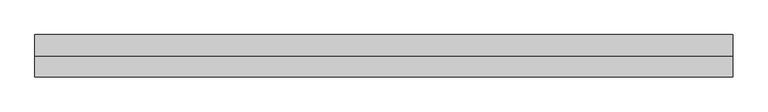
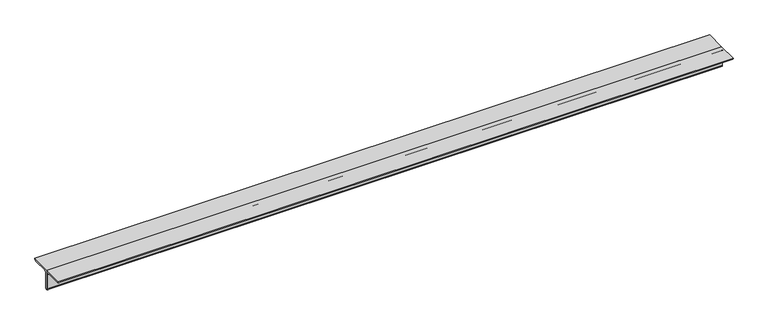
"""IFC4 building model written with IfcOpenShell, lengths in millimetres: member geometry, 0123_Steel Framing_2Ls-KSD3502 : H_SB_AR_S03_2Ls-130x130x12_HBR4."""

import ifcopenshell
import ifcopenshell.guid

model = None  # the IFC model being written
_history = None  # IfcOwnerHistory: only IFC2X3 demands one
_inside = {}  # id of a spatial element -> (the spatial element, [elements in it])
_under = {}  # id of a project, library or spatial element -> (it, [spatial elements below it])
_declared = {}  # id of a project -> (the project, [libraries it declares])
_typed = {}  # id of a type object -> (the type object, [elements of that type])
_made_of = {}  # id of a material, layer set ... -> (it, [elements and type objects made of it])


def new_model(schema):
    """Start an empty IFC model of exactly this schema.

    Asked for "IFC4X3", IfcOpenShell would pick the latest addendum, in which some entities
    have other attributes; the version numbers below select the first issue.
    IFC2X3 requires an IfcOwnerHistory on every rooted entity: one is made here for all.
    """
    global model, _history
    if schema == "IFC4X3":
        model = ifcopenshell.file(schema_version=(4, 3, 0, 0))
    else:
        model = ifcopenshell.file(schema=schema)
    _inside.clear()
    _under.clear()
    _declared.clear()
    _typed.clear()
    _made_of.clear()
    _history = None
    if model.schema == "IFC2X3":
        org = make("IfcOrganization", Name="unknown")
        user = make(
            "IfcPersonAndOrganization",
            ThePerson=make("IfcPerson", FamilyName="unknown"),
            TheOrganization=org,
        )
        app = make(
            "IfcApplication",
            ApplicationDeveloper=org,
            Version="unknown",
            ApplicationFullName="unknown",
            ApplicationIdentifier="unknown",
        )
        _history = make(
            "IfcOwnerHistory",
            OwningUser=user,
            OwningApplication=app,
            ChangeAction="ADDED",
            CreationDate=0,
        )
    return model


def make(cls, **values):
    """One entity of the class cls with the attributes given. An attribute that is None is left unset."""
    return model.create_entity(
        cls, **{name: value for name, value in values.items() if value is not None}
    )


def rooted(cls, **values):
    """An entity with a GlobalId (a new one), such as an element, a storey or a relation."""
    return make(cls, GlobalId=ifcopenshell.guid.new(), OwnerHistory=_history, **values)


def si_unit(unit_type, name, prefix=None):
    """IfcSIUnit, for example si_unit("LENGTHUNIT", "METRE", prefix="MILLI")."""
    return make("IfcSIUnit", UnitType=unit_type, Prefix=prefix, Name=name)


def assignment(units):
    """IfcUnitAssignment: the units of a project."""
    return None if units is None else make("IfcUnitAssignment", Units=units)


def point(xyz):
    """IfcCartesianPoint."""
    return None if xyz is None else make("IfcCartesianPoint", Coordinates=xyz)


def direction(xyz):
    """IfcDirection."""
    return None if xyz is None else make("IfcDirection", DirectionRatios=xyz)


def frame(location, z_axis=None, x_axis=None):
    """IfcAxis2Placement3D, a coordinate frame: its origin and axes. An axis left out is left unset."""
    return make(
        "IfcAxis2Placement3D",
        Location=point(location),
        Axis=direction(z_axis),
        RefDirection=direction(x_axis),
    )


def frame_2d(location, x_axis=None):
    """IfcAxis2Placement2D, a coordinate frame in the plane: its origin and x axis."""
    return make(
        "IfcAxis2Placement2D", Location=point(location), RefDirection=direction(x_axis)
    )


def origin():
    """The frame at (0, 0, 0) with its axes left unset."""
    return frame((0.0, 0.0, 0.0))


def place(relative_to, where):
    """IfcLocalPlacement: puts the frame where relative to a parent placement (None: the world)."""
    return make(
        "IfcLocalPlacement", PlacementRelTo=relative_to, RelativePlacement=where
    )


def context(
    kind, dimensions, precision=None, world=None, true_north=None, identifier=None
):
    """IfcGeometricRepresentationContext, for example the 3D "Model" context."""
    return make(
        "IfcGeometricRepresentationContext",
        ContextIdentifier=identifier,
        ContextType=kind,
        CoordinateSpaceDimension=dimensions,
        Precision=precision,
        WorldCoordinateSystem=world,
        TrueNorth=true_north,
    )


def project(units=None, contexts=None):
    """IfcProject with its units and contexts."""
    return rooted(
        "IfcProject",
        Name="project",
        RepresentationContexts=contexts,
        UnitsInContext=assignment(units),
    )


def spatial(cls, under=None, at=None, **own):
    """A site, building, storey or space (cls), placed at a placement, below another one or the project."""
    s = rooted(cls, ObjectPlacement=at, **own)
    if under is not None:
        _under.setdefault(under.id(), (under, []))[1].append(s)
    return s


def polyline(points):
    """IfcPolyline through the points."""
    return make("IfcPolyline", Points=[point(p) for p in points])


def circle_curve(where, radius):
    """IfcCircle in the frame where."""
    return make("IfcCircle", Position=where, Radius=radius)


def trimmed(basis, trim1, trim2, sense, master):
    """IfcTrimmedCurve: the piece of a basis curve between two trims."""
    return make(
        "IfcTrimmedCurve",
        BasisCurve=basis,
        Trim1=trim1,
        Trim2=trim2,
        SenseAgreement=sense,
        MasterRepresentation=master,
    )


def segment(curve, same_sense, transition):
    """IfcCompositeCurveSegment."""
    return make(
        "IfcCompositeCurveSegment",
        Transition=transition,
        SameSense=same_sense,
        ParentCurve=curve,
    )


def composite_curve(segments, self_intersect=None):
    """IfcCompositeCurve: segments joined end to end."""
    return make("IfcCompositeCurve", Segments=segments, SelfIntersect=self_intersect)


def outline(outer, holes=None, kind="AREA"):
    """IfcArbitraryClosedProfileDef: a profile drawn as a closed curve; with holes, ...WithVoids."""
    if holes is None:
        return make("IfcArbitraryClosedProfileDef", ProfileType=kind, OuterCurve=outer)
    return make(
        "IfcArbitraryProfileDefWithVoids",
        ProfileType=kind,
        OuterCurve=outer,
        InnerCurves=holes,
    )


def extrude(swept, where, along, depth):
    """IfcExtrudedAreaSolid: the profile swept, set in the frame where, extruded along a direction by depth."""
    return make(
        "IfcExtrudedAreaSolid",
        SweptArea=swept,
        Position=where,
        ExtrudedDirection=direction(along),
        Depth=depth,
    )


def shape(context_of_items, identifier, shape_type, items):
    """IfcShapeRepresentation: the items that make up one representation, for example the "Body"."""
    return make(
        "IfcShapeRepresentation",
        ContextOfItems=context_of_items,
        RepresentationIdentifier=identifier,
        RepresentationType=shape_type,
        Items=items,
    )


def source(mapping_origin, context_of_items, identifier, shape_type, items):
    """IfcRepresentationMap: a shape defined once, which mapped items show again and again."""
    return make(
        "IfcRepresentationMap",
        MappingOrigin=mapping_origin,
        MappedRepresentation=shape(context_of_items, identifier, shape_type, items),
    )


def transform(
    local_origin,
    x_axis=None,
    y_axis=None,
    z_axis=None,
    scale=None,
    scale2=None,
    scale3=None,
    uniform=True,
):
    """IfcCartesianTransformationOperator3D, or its non-uniform kind. x_axis, y_axis, z_axis: its Axis1, 2, 3."""
    if uniform:
        return make(
            "IfcCartesianTransformationOperator3D",
            Axis1=direction(x_axis),
            Axis2=direction(y_axis),
            LocalOrigin=point(local_origin),
            Scale=scale,
            Axis3=direction(z_axis),
        )
    return make(
        "IfcCartesianTransformationOperator3DnonUniform",
        Axis1=direction(x_axis),
        Axis2=direction(y_axis),
        LocalOrigin=point(local_origin),
        Scale=scale,
        Axis3=direction(z_axis),
        Scale2=scale2,
        Scale3=scale3,
    )


def mapped(mapping_source, mapping_target):
    """IfcMappedItem: shows the shape of a source again, moved by a transform."""
    return make(
        "IfcMappedItem", MappingSource=mapping_source, MappingTarget=mapping_target
    )


def made_of(thing, what):
    """Note that an element or type object is made of a material, layer set ...; save() writes the relation."""
    if what is not None:
        _made_of.setdefault(what.id(), (what, []))[1].append(thing)
    return thing


def element(
    cls,
    number,
    at=None,
    inside=None,
    cuts=None,
    type_object=None,
    material=None,
    context=None,
    identifier="Body",
    shape_type=None,
    held_by="IfcProductDefinitionShape",
    body=None,
    shapes=None,
    **own,
):
    """One element of the class cls, such as IfcWall. Its Tag is "e" and its number.

    at: its placement. inside: the storey or other place that contains it. cuts: it is an
    opening in that element (IfcRelVoidsElement). A single representation is given by context,
    identifier, shape_type and body (its items); several are given by shapes. held_by: the class
    of the entity that holds the representations. save() writes the other relations.
    """
    e = rooted(cls, Tag="e%d" % number, ObjectPlacement=at, **own)
    if body is not None:
        shapes = [shape(context, identifier, shape_type, body)]
    if shapes is not None:
        e.Representation = make(held_by, Representations=shapes)
    if inside is not None:
        _inside.setdefault(inside.id(), (inside, []))[1].append(e)
    if cuts is not None:
        rooted(
            "IfcRelVoidsElement", RelatingBuildingElement=cuts, RelatedOpeningElement=e
        )
    if type_object is not None:
        _typed.setdefault(type_object.id(), (type_object, []))[1].append(e)
    return made_of(e, material)


def aggregate(whole, parts):
    """IfcRelAggregates: a whole, such as a stair, and the parts it consists of."""
    return rooted("IfcRelAggregates", RelatingObject=whole, RelatedObjects=parts)


def save(model, path):
    """Write the relations noted so far, then the file.

    IfcRelAggregates (storeys below a building ...), IfcRelContainedInSpatialStructure (elements
    in a storey), IfcRelDefinesByType, IfcRelAssociatesMaterial and IfcRelDeclares: one each for
    every whole, place, type object, material and project.
    """
    for whole, parts in _under.values():
        aggregate(whole, parts)
    for where, things in _inside.values():
        rooted(
            "IfcRelContainedInSpatialStructure",
            RelatedElements=things,
            RelatingStructure=where,
        )
    for kind, things in _typed.values():
        rooted("IfcRelDefinesByType", RelatedObjects=things, RelatingType=kind)
    for what, things in _made_of.values():
        rooted("IfcRelAssociatesMaterial", RelatedObjects=things, RelatingMaterial=what)
    for by, libraries in _declared.values():
        rooted("IfcRelDeclares", RelatingContext=by, RelatedDefinitions=libraries)
    model.write(path)


def member_b79bbe70(model_context):
    return source(origin(), model_context, "Body", "SweptSolid", [
        extrude(outline(composite_curve([segment(polyline([(0.0, 36.4), (130.0, 36.4)]), True, "CONTINUOUS"), segment(trimmed(circle_curve(frame_2d((118.0, 36.4)), 12.0), [point((130.0, 36.4))], [point((118.0, 24.4))], False, "CARTESIAN"), True, "CONTINUOUS"), segment(polyline([(118.0, 24.4), (24.0, 24.4)]), True, "CONTINUOUS"), segment(trimmed(circle_curve(frame_2d((24.0, 12.4)), 12.0), [point((24.0, 24.4))], [point((12.0, 12.4))], True, "CARTESIAN"), True, "CONTINUOUS"), segment(polyline([(12.0, 12.4), (12.0, -81.6)]), True, "CONTINUOUS"), segment(trimmed(circle_curve(frame_2d((0.0, -81.6)), 12.0), [point((12.0, -81.6))], [point((0.0, -93.6))], False, "CARTESIAN"), True, "CONTINUOUS"), segment(polyline([(0.0, -93.6), (0.0, 36.4)]), True, "CONTINUOUS")], self_intersect=False)), frame((-2078.9666667, 0.0, 0.0), z_axis=(1.0, 0.0, 0.0), x_axis=(0.0, 1.0, 0.0)), (0.0, 0.0, 1.0), 4294.8666667),
        extrude(outline(composite_curve([segment(polyline([(0.0, 36.4), (0.0, -93.6)]), True, "CONTINUOUS"), segment(trimmed(circle_curve(frame_2d((0.0, -81.6)), 12.0), [point((0.0, -93.6))], [point((-12.0, -81.6))], False, "CARTESIAN"), True, "CONTINUOUS"), segment(polyline([(-12.0, -81.6), (-12.0, 12.4)]), True, "CONTINUOUS"), segment(trimmed(circle_curve(frame_2d((-24.0, 12.4)), 12.0), [point((-12.0, 12.4))], [point((-24.0, 24.4))], True, "CARTESIAN"), True, "CONTINUOUS"), segment(polyline([(-24.0, 24.4), (-118.0, 24.4)]), True, "CONTINUOUS"), segment(trimmed(circle_curve(frame_2d((-118.0, 36.4)), 12.0), [point((-118.0, 24.4))], [point((-130.0, 36.4))], False, "CARTESIAN"), True, "CONTINUOUS"), segment(polyline([(-130.0, 36.4), (0.0, 36.4)]), True, "CONTINUOUS")], self_intersect=False)), frame((-2078.9666667, 0.0, 0.0), z_axis=(1.0, 0.0, 0.0), x_axis=(0.0, 1.0, 0.0)), (0.0, 0.0, 1.0), 4294.8666667),
    ])


if __name__ == "__main__":
    model = new_model("IFC4")
    model_context = context("Model", 3, world=origin())
    ifc_project = project(units=[si_unit("LENGTHUNIT", "METRE", prefix="MILLI")], contexts=[model_context])
    site = spatial("IfcSite", under=ifc_project)
    building = spatial("IfcBuilding", under=site)
    placement = place(None, origin())
    member_shape = member_b79bbe70(model_context)
    element("IfcMember", 1, ObjectType="0123_Steel Framing_2Ls-KSD3502 : H_SB_AR_S03_2Ls-130x130x12_HBR4", at=placement, inside=building, context=model_context, shape_type="MappedRepresentation", body=[
        mapped(member_shape, transform((0.0, 0.0, 0.0), x_axis=(1.0, 0.0, 0.0), y_axis=(0.0, 1.0, 0.0), z_axis=(0.0, 0.0, 1.0))),
    ])
    save(model, "model.ifc")

# Revit data of these elements
# Type "0123_Steel Framing_2Ls-KSD3502 : H_SB_AR_S03_2Ls-130x130x12_HBR4"
#   Assembly Code = "B10"
#   Legs = "SLBB"
#   W = 8.97
#   Perimeter = 1.04 m²/m
#   Nominal Weight = 46.80 kgf/m
#   Length [instance default] = 1000 mm
#   Space = 0 mm
#   b = 130 mm
#   d = 130 mm
#   t = 12 mm
#   y = 36.4 mm
#   A = 0.005952 m²
#   Structural Material [instance default] = Steel ASTM A36
# Element 1 (IfcMember, "0123_Steel Framing_2Ls-KSD3502 : H_SB_AR_S03_2Ls-130x130x12_HBR4")
#   Structural Material = Steel, 45-345
#   Materials on its faces: "Steel, 45-345"
# Materials
#   "Steel ASTM A36": class "Metal", colour RGB 199 199 199, transparency 0, Description = "Structural steel, ASTM A36 Grade B, mill finish", Cost = 0
#   "Steel, 45-345": class "Metal", colour RGB 189 187 185, transparency 0, Description = "Steel 345 MPa", Cost = 0
